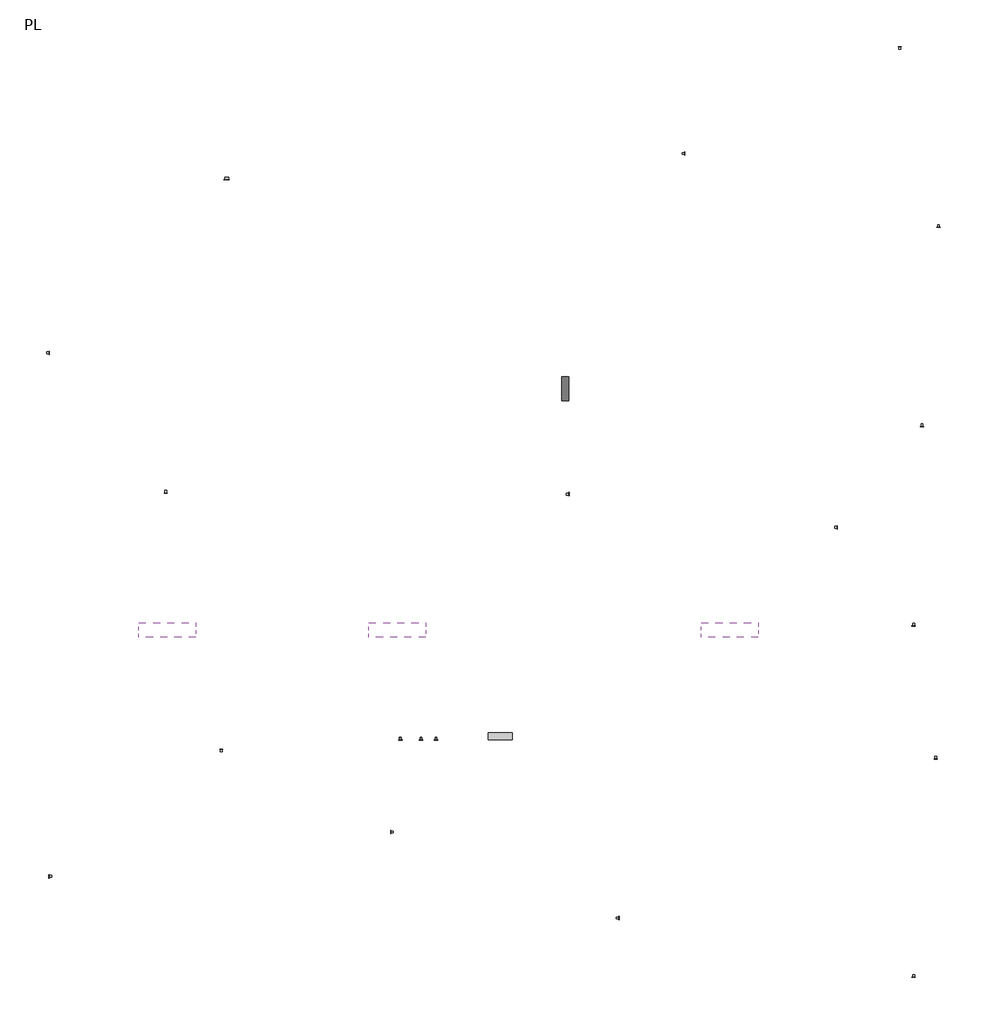
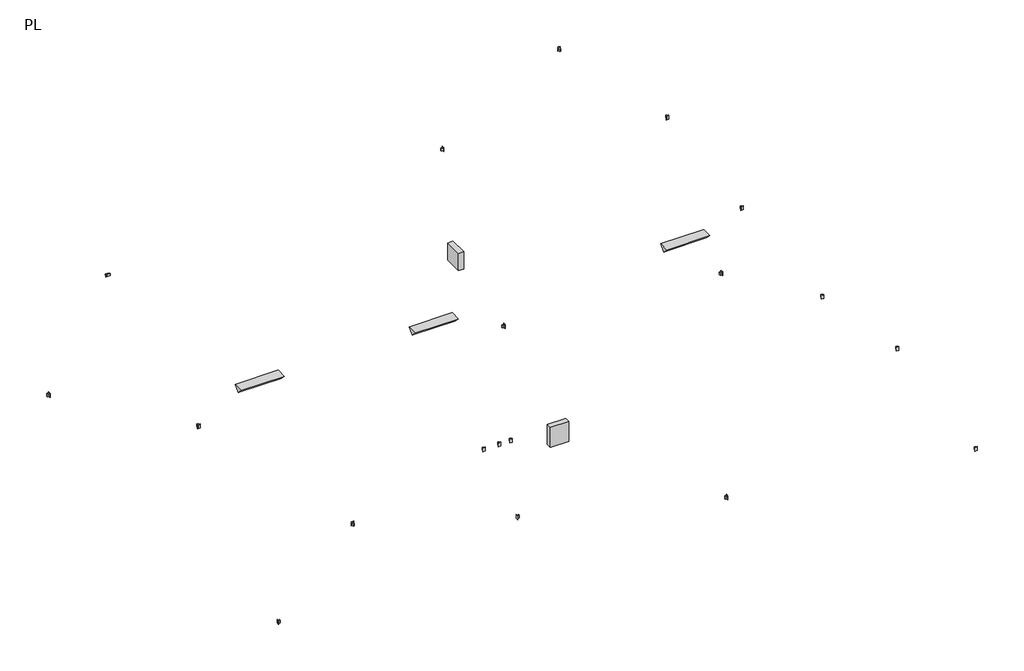
# One storey: 18 proxies, 3 light fixtures, 3 switching devices.
"""IFC4 building model written with IfcOpenShell, lengths in millimetres."""

import ifcopenshell
import ifcopenshell.guid

model = None  # the IFC model being written
_history = None  # IfcOwnerHistory: only IFC2X3 demands one
_inside = {}  # id of a spatial element -> (the spatial element, [elements in it])
_under = {}  # id of a project, library or spatial element -> (it, [spatial elements below it])
_declared = {}  # id of a project -> (the project, [libraries it declares])
_typed = {}  # id of a type object -> (the type object, [elements of that type])
_made_of = {}  # id of a material, layer set ... -> (it, [elements and type objects made of it])


def new_model(schema):
    """Start an empty IFC model of exactly this schema.

    Asked for "IFC4X3", IfcOpenShell would pick the latest addendum, in which some entities
    have other attributes; the version numbers below select the first issue.
    IFC2X3 requires an IfcOwnerHistory on every rooted entity: one is made here for all.
    """
    global model, _history
    if schema == "IFC4X3":
        model = ifcopenshell.file(schema_version=(4, 3, 0, 0))
    else:
        model = ifcopenshell.file(schema=schema)
    _inside.clear()
    _under.clear()
    _declared.clear()
    _typed.clear()
    _made_of.clear()
    _history = None
    if model.schema == "IFC2X3":
        org = make("IfcOrganization", Name="unknown")
        user = make(
            "IfcPersonAndOrganization",
            ThePerson=make("IfcPerson", FamilyName="unknown"),
            TheOrganization=org,
        )
        app = make(
            "IfcApplication",
            ApplicationDeveloper=org,
            Version="unknown",
            ApplicationFullName="unknown",
            ApplicationIdentifier="unknown",
        )
        _history = make(
            "IfcOwnerHistory",
            OwningUser=user,
            OwningApplication=app,
            ChangeAction="ADDED",
            CreationDate=0,
        )
    return model


def make(cls, **values):
    """One entity of the class cls with the attributes given. An attribute that is None is left unset."""
    return model.create_entity(
        cls, **{name: value for name, value in values.items() if value is not None}
    )


def rooted(cls, **values):
    """An entity with a GlobalId (a new one), such as an element, a storey or a relation."""
    return make(cls, GlobalId=ifcopenshell.guid.new(), OwnerHistory=_history, **values)


def si_unit(unit_type, name, prefix=None):
    """IfcSIUnit, for example si_unit("LENGTHUNIT", "METRE", prefix="MILLI")."""
    return make("IfcSIUnit", UnitType=unit_type, Prefix=prefix, Name=name)


def assignment(units):
    """IfcUnitAssignment: the units of a project."""
    return None if units is None else make("IfcUnitAssignment", Units=units)


def point(xyz):
    """IfcCartesianPoint."""
    return None if xyz is None else make("IfcCartesianPoint", Coordinates=xyz)


def direction(xyz):
    """IfcDirection."""
    return None if xyz is None else make("IfcDirection", DirectionRatios=xyz)


def frame(location, z_axis=None, x_axis=None):
    """IfcAxis2Placement3D, a coordinate frame: its origin and axes. An axis left out is left unset."""
    return make(
        "IfcAxis2Placement3D",
        Location=point(location),
        Axis=direction(z_axis),
        RefDirection=direction(x_axis),
    )


def origin():
    """The frame at (0, 0, 0) with its axes left unset."""
    return frame((0.0, 0.0, 0.0))


def origin_with_axes():
    """The frame at (0, 0, 0) with the z axis (0, 0, 1) and the x axis (1, 0, 0) written out."""
    return frame((0.0, 0.0, 0.0), z_axis=(0.0, 0.0, 1.0), x_axis=(1.0, 0.0, 0.0))


def place(relative_to, where):
    """IfcLocalPlacement: puts the frame where relative to a parent placement (None: the world)."""
    return make(
        "IfcLocalPlacement", PlacementRelTo=relative_to, RelativePlacement=where
    )


def context(
    kind, dimensions, precision=None, world=None, true_north=None, identifier=None
):
    """IfcGeometricRepresentationContext, for example the 3D "Model" context."""
    return make(
        "IfcGeometricRepresentationContext",
        ContextIdentifier=identifier,
        ContextType=kind,
        CoordinateSpaceDimension=dimensions,
        Precision=precision,
        WorldCoordinateSystem=world,
        TrueNorth=true_north,
    )


def project(units=None, contexts=None):
    """IfcProject with its units and contexts."""
    return rooted(
        "IfcProject",
        Name="project",
        RepresentationContexts=contexts,
        UnitsInContext=assignment(units),
    )


def spatial(cls, under=None, at=None, **own):
    """A site, building, storey or space (cls), placed at a placement, below another one or the project."""
    s = rooted(cls, ObjectPlacement=at, **own)
    if under is not None:
        _under.setdefault(under.id(), (under, []))[1].append(s)
    return s


def polyline(points):
    """IfcPolyline through the points."""
    return make("IfcPolyline", Points=[point(p) for p in points])


def outline(outer, holes=None, kind="AREA"):
    """IfcArbitraryClosedProfileDef: a profile drawn as a closed curve; with holes, ...WithVoids."""
    if holes is None:
        return make("IfcArbitraryClosedProfileDef", ProfileType=kind, OuterCurve=outer)
    return make(
        "IfcArbitraryProfileDefWithVoids",
        ProfileType=kind,
        OuterCurve=outer,
        InnerCurves=holes,
    )


def extrude(swept, where, along, depth):
    """IfcExtrudedAreaSolid: the profile swept, set in the frame where, extruded along a direction by depth."""
    return make(
        "IfcExtrudedAreaSolid",
        SweptArea=swept,
        Position=where,
        ExtrudedDirection=direction(along),
        Depth=depth,
    )


def shape(context_of_items, identifier, shape_type, items):
    """IfcShapeRepresentation: the items that make up one representation, for example the "Body"."""
    return make(
        "IfcShapeRepresentation",
        ContextOfItems=context_of_items,
        RepresentationIdentifier=identifier,
        RepresentationType=shape_type,
        Items=items,
    )


def source(mapping_origin, context_of_items, identifier, shape_type, items):
    """IfcRepresentationMap: a shape defined once, which mapped items show again and again."""
    return make(
        "IfcRepresentationMap",
        MappingOrigin=mapping_origin,
        MappedRepresentation=shape(context_of_items, identifier, shape_type, items),
    )


def transform(
    local_origin,
    x_axis=None,
    y_axis=None,
    z_axis=None,
    scale=None,
    scale2=None,
    scale3=None,
    uniform=True,
):
    """IfcCartesianTransformationOperator3D, or its non-uniform kind. x_axis, y_axis, z_axis: its Axis1, 2, 3."""
    if uniform:
        return make(
            "IfcCartesianTransformationOperator3D",
            Axis1=direction(x_axis),
            Axis2=direction(y_axis),
            LocalOrigin=point(local_origin),
            Scale=scale,
            Axis3=direction(z_axis),
        )
    return make(
        "IfcCartesianTransformationOperator3DnonUniform",
        Axis1=direction(x_axis),
        Axis2=direction(y_axis),
        LocalOrigin=point(local_origin),
        Scale=scale,
        Axis3=direction(z_axis),
        Scale2=scale2,
        Scale3=scale3,
    )


def mapped(mapping_source, mapping_target):
    """IfcMappedItem: shows the shape of a source again, moved by a transform."""
    return make(
        "IfcMappedItem", MappingSource=mapping_source, MappingTarget=mapping_target
    )


def made_of(thing, what):
    """Note that an element or type object is made of a material, layer set ...; save() writes the relation."""
    if what is not None:
        _made_of.setdefault(what.id(), (what, []))[1].append(thing)
    return thing


def element(
    cls,
    number,
    at=None,
    inside=None,
    cuts=None,
    type_object=None,
    material=None,
    context=None,
    identifier="Body",
    shape_type=None,
    held_by="IfcProductDefinitionShape",
    body=None,
    shapes=None,
    **own,
):
    """One element of the class cls, such as IfcWall. Its Tag is "e" and its number.

    at: its placement. inside: the storey or other place that contains it. cuts: it is an
    opening in that element (IfcRelVoidsElement). A single representation is given by context,
    identifier, shape_type and body (its items); several are given by shapes. held_by: the class
    of the entity that holds the representations. save() writes the other relations.
    """
    e = rooted(cls, Tag="e%d" % number, ObjectPlacement=at, **own)
    if body is not None:
        shapes = [shape(context, identifier, shape_type, body)]
    if shapes is not None:
        e.Representation = make(held_by, Representations=shapes)
    if inside is not None:
        _inside.setdefault(inside.id(), (inside, []))[1].append(e)
    if cuts is not None:
        rooted(
            "IfcRelVoidsElement", RelatingBuildingElement=cuts, RelatedOpeningElement=e
        )
    if type_object is not None:
        _typed.setdefault(type_object.id(), (type_object, []))[1].append(e)
    return made_of(e, material)


def aggregate(whole, parts):
    """IfcRelAggregates: a whole, such as a stair, and the parts it consists of."""
    return rooted("IfcRelAggregates", RelatingObject=whole, RelatedObjects=parts)


def save(model, path):
    """Write the relations noted so far, then the file.

    IfcRelAggregates (storeys below a building ...), IfcRelContainedInSpatialStructure (elements
    in a storey), IfcRelDefinesByType, IfcRelAssociatesMaterial and IfcRelDeclares: one each for
    every whole, place, type object, material and project.
    """
    for whole, parts in _under.values():
        aggregate(whole, parts)
    for where, things in _inside.values():
        rooted(
            "IfcRelContainedInSpatialStructure",
            RelatedElements=things,
            RelatingStructure=where,
        )
    for kind, things in _typed.values():
        rooted("IfcRelDefinesByType", RelatedObjects=things, RelatingType=kind)
    for what, things in _made_of.values():
        rooted("IfcRelAssociatesMaterial", RelatedObjects=things, RelatingMaterial=what)
    for by, libraries in _declared.values():
        rooted("IfcRelDeclares", RelatingContext=by, RelatedDefinitions=libraries)
    model.write(path)


def m_duplex_receptacle_standard_10251bba(model_context):
    return source(origin(), model_context, "Body", "SweptSolid", [
        extrude(outline(polyline([(19.05, 38.1), (19.05, -38.1), (-19.05, -38.1), (-19.05, 38.1), (19.05, 38.1)])), frame((0.0, 0.0, -53.975), z_axis=(0.0, 0.0, 1.0), x_axis=(1.0, 0.0, 0.0)), (0.0, 0.0, 1.0), 53.975),
        extrude(outline(polyline([(34.925, 57.15), (34.925, -57.15), (-34.925, -57.15), (-34.925, 57.15), (34.925, 57.15)])), origin_with_axes(), (0.0, 0.0, 1.0), 4.7625),
    ])


def m_lighting_and_appliance_panelboard_208v_mcb_100_a_1c5cc82c(model_context):
    return source(origin(), model_context, "Body", "SweptSolid", [
        extrude(outline(polyline([(349.2594706, 55.9943297), (349.2594706, -528.2056703), (-158.7405294, -528.2056703), (-158.7405294, 55.9943297), (349.2594706, 55.9943297)])), frame((0.0, 0.0, -146.1), z_axis=(0.0, 0.0, 1.0), x_axis=(1.0, 0.0, 0.0)), (0.0, 0.0, 1.0), 146.1),
    ])


def m_lighting_and_appliance_panelboard_208v_mlo_100_a_deb79597(model_context):
    return source(origin(), model_context, "Body", "SweptSolid", [
        extrude(outline(polyline([(254.0, -165.1), (254.0, -673.1), (-254.0, -673.1), (-254.0, -165.1), (254.0, -165.1)])), frame((0.0, 0.0, -146.1), z_axis=(0.0, 0.0, 1.0), x_axis=(1.0, 0.0, 0.0)), (0.0, 0.0, 1.0), 146.1),
    ])


def m_plain_recessed_lighting_fixture_300x1200_120_e46e8774(model_context):
    return source(origin(), model_context, "Body", "SweptSolid", [
        extrude(outline(polyline([(-300.0, 0.0), (0.0, 0.0), (-150.0, -150.0), (-300.0, 0.0)])), frame((0.0, 0.0, 0.0), z_axis=(1.0, 0.0, 0.0), x_axis=(0.0, 1.0, 0.0)), (0.0, 0.0, 1.0), 1200.0),
    ])


model = new_model("IFC4")

# Units and contexts
model_context = context("Model", 3, world=origin())
ifc_project = project(units=[si_unit("LENGTHUNIT", "METRE", prefix="MILLI")], contexts=[model_context])

# Site, building, storey
site = spatial("IfcSite", under=ifc_project)
building = spatial("IfcBuilding", under=site)
storey = spatial("IfcBuildingStorey", under=building, Name="PL", Elevation=500.0)

# Proxies
placement = place(None, origin())
m_duplex_receptacle_standard_shape = m_duplex_receptacle_standard_10251bba(model_context)
element("IfcBuildingElementProxy", 1, Name="M_Duplex Receptacle : Standard", ObjectType="M_Duplex Receptacle : Standard", at=placement, inside=storey, context=model_context, shape_type="MappedRepresentation", body=[
    mapped(m_duplex_receptacle_standard_shape, transform((-11924.1082979, -105.8587328, 960.0), x_axis=(1.0, 0.0, 0.0), y_axis=(0.0, 0.0, 1.0), z_axis=(0.0, -1.0, 0.0))),
])
element("IfcBuildingElementProxy", 2, Name="M_Duplex Receptacle : Standard", ObjectType="M_Duplex Receptacle : Standard", at=placement, inside=storey, context=model_context, shape_type="MappedRepresentation", body=[
    mapped(m_duplex_receptacle_standard_shape, transform((-10757.1359856, -5505.8587328, 960.0), x_axis=(-1.0, 0.0, 0.0), y_axis=(0.0, 0.0, 1.0), z_axis=(0.0, 1.0, 0.0))),
])
element("IfcBuildingElementProxy", 3, Name="M_Duplex Receptacle : Standard", ObjectType="M_Duplex Receptacle : Standard", at=placement, inside=storey, context=model_context, shape_type="MappedRepresentation", body=[
    mapped(m_duplex_receptacle_standard_shape, transform((-14381.6781998, -8181.5416269, 960.0), x_axis=(0.0, -1.0, 0.0), y_axis=(0.0, 0.0, 1.0), z_axis=(-1.0, 0.0, 0.0))),
])
element("IfcBuildingElementProxy", 4, Name="M_Duplex Receptacle : Standard", ObjectType="M_Duplex Receptacle : Standard", at=placement, inside=storey, context=model_context, shape_type="MappedRepresentation", body=[
    mapped(m_duplex_receptacle_standard_shape, transform((2218.3218002, -829.616059, 960.0), x_axis=(0.0, 1.0, 0.0), y_axis=(0.0, 0.0, 1.0), z_axis=(1.0, 0.0, 0.0))),
])
element("IfcBuildingElementProxy", 5, Name="M_Duplex Receptacle : Standard", ObjectType="M_Duplex Receptacle : Standard", at=placement, inside=storey, context=model_context, shape_type="MappedRepresentation", body=[
    mapped(m_duplex_receptacle_standard_shape, transform((-14381.6781998, 2846.3467249, 960.0), x_axis=(0.0, -1.0, 0.0), y_axis=(0.0, 0.0, -1.0), z_axis=(1.0, 0.0, 0.0))),
])
element("IfcBuildingElementProxy", 6, Name="M_Duplex Receptacle : Standard", ObjectType="M_Duplex Receptacle : Standard", at=placement, inside=storey, context=model_context, shape_type="MappedRepresentation", body=[
    mapped(m_duplex_receptacle_standard_shape, transform((4355.1554595, 5494.1412672, 960.0), x_axis=(1.0, 0.0, 0.0), y_axis=(0.0, 0.0, 1.0), z_axis=(0.0, -1.0, 0.0))),
])
element("IfcBuildingElementProxy", 7, Name="M_Duplex Receptacle : Standard", ObjectType="M_Duplex Receptacle : Standard", at=placement, inside=storey, context=model_context, shape_type="MappedRepresentation", body=[
    mapped(m_duplex_receptacle_standard_shape, transform((3538.2748408, 9294.1412672, 960.0), x_axis=(-1.0, 0.0, 0.0), y_axis=(0.0, 0.0, 1.0), z_axis=(0.0, 1.0, 0.0))),
])
element("IfcBuildingElementProxy", 8, Name="M_Duplex Receptacle : Standard", ObjectType="M_Duplex Receptacle : Standard", at=placement, inside=storey, context=model_context, shape_type="MappedRepresentation", body=[
    mapped(m_duplex_receptacle_standard_shape, transform((3830.0179189, -2905.8587328, 960.0), x_axis=(1.0, 0.0, 0.0), y_axis=(0.0, 0.0, 1.0), z_axis=(0.0, -1.0, 0.0))),
])
element("IfcBuildingElementProxy", 9, Name="M_Duplex Receptacle : Standard", ObjectType="M_Duplex Receptacle : Standard", at=placement, inside=storey, context=model_context, shape_type="MappedRepresentation", body=[
    mapped(m_duplex_receptacle_standard_shape, transform((4005.0637658, 1294.1412672, 960.0), x_axis=(1.0, 0.0, 0.0), y_axis=(0.0, 0.0, 1.0), z_axis=(0.0, -1.0, 0.0))),
])
element("IfcBuildingElementProxy", 10, Name="M_Duplex Receptacle : Standard", ObjectType="M_Duplex Receptacle : Standard", at=placement, inside=storey, context=model_context, shape_type="MappedRepresentation", body=[
    mapped(m_duplex_receptacle_standard_shape, transform((4296.8068439, -5705.8587328, 960.0), x_axis=(1.0, 0.0, 0.0), y_axis=(0.0, 0.0, 1.0), z_axis=(0.0, -1.0, 0.0))),
])
element("IfcBuildingElementProxy", 11, Name="M_Duplex Receptacle : Standard", ObjectType="M_Duplex Receptacle : Standard", at=placement, inside=storey, context=model_context, shape_type="MappedRepresentation", body=[
    mapped(m_duplex_receptacle_standard_shape, transform((3830.0179189, -10305.8587328, 960.0), x_axis=(1.0, 0.0, 0.0), y_axis=(0.0, 0.0, 1.0), z_axis=(0.0, -1.0, 0.0))),
])
element("IfcBuildingElementProxy", 12, Name="M_Duplex Receptacle : Standard", ObjectType="M_Duplex Receptacle : Standard", at=placement, inside=storey, context=model_context, shape_type="MappedRepresentation", body=[
    mapped(m_duplex_receptacle_standard_shape, transform((-2381.6781998, -9056.7708611, 960.0), x_axis=(0.0, -1.0, 0.0), y_axis=(0.0, 0.0, -1.0), z_axis=(1.0, 0.0, 0.0))),
])
element("IfcBuildingElementProxy", 13, Name="M_Duplex Receptacle : Standard", ObjectType="M_Duplex Receptacle : Standard", at=placement, inside=storey, context=model_context, shape_type="MappedRepresentation", body=[
    mapped(m_duplex_receptacle_standard_shape, transform((-7181.6781998, -7247.963777, 960.0), x_axis=(0.0, -1.0, 0.0), y_axis=(0.0, 0.0, 1.0), z_axis=(-1.0, 0.0, 0.0))),
])
element("IfcBuildingElementProxy", 14, Name="M_Duplex Receptacle : Standard", ObjectType="M_Duplex Receptacle : Standard", at=placement, inside=storey, context=model_context, shape_type="MappedRepresentation", body=[
    mapped(m_duplex_receptacle_standard_shape, transform((-10640.4387543, 6494.1412672, 960.0), x_axis=(0.0, 0.0, 1.0), y_axis=(-1.0, 0.0, 0.0), z_axis=(0.0, -1.0, 0.0))),
])
element("IfcBuildingElementProxy", 15, Name="M_Duplex Receptacle : Standard", ObjectType="M_Duplex Receptacle : Standard", at=placement, inside=storey, context=model_context, shape_type="MappedRepresentation", body=[
    mapped(m_duplex_receptacle_standard_shape, transform((-991.6781998, 7047.4470494, 960.0), x_axis=(0.0, 1.0, 0.0), y_axis=(0.0, 0.0, 1.0), z_axis=(1.0, 0.0, 0.0))),
])
element("IfcBuildingElementProxy", 16, Name="M_Duplex Receptacle : Standard", ObjectType="M_Duplex Receptacle : Standard", at=placement, inside=storey, context=model_context, shape_type="MappedRepresentation", body=[
    mapped(m_duplex_receptacle_standard_shape, transform((-3431.6781998, -129.4326716, 960.0), x_axis=(0.0, 1.0, 0.0), y_axis=(0.0, 0.0, 1.0), z_axis=(1.0, 0.0, 0.0))),
])
m_lighting_and_appliance_panelboard_208v_mcb_100_a_shape = m_lighting_and_appliance_panelboard_208v_mcb_100_a_1c5cc82c(model_context)
element("IfcBuildingElementProxy", 17, Name="M_Lighting and Appliance Panelboard - 208V MCB : 100 A", ObjectType="M_Lighting and Appliance Panelboard - 208V MCB : 100 A", at=placement, inside=storey, context=model_context, shape_type="MappedRepresentation", body=[
    mapped(m_lighting_and_appliance_panelboard_208v_mcb_100_a_shape, transform((-4974.3445292, -5305.8587328, 1644.0056703), x_axis=(1.0, 0.0, 0.0), y_axis=(0.0, 0.0, 1.0), z_axis=(0.0, -1.0, 0.0))),
])
m_lighting_and_appliance_panelboard_208v_mlo_100_a_shape = m_lighting_and_appliance_panelboard_208v_mlo_100_a_deb79597(model_context)
element("IfcBuildingElementProxy", 18, Name="M_Lighting and Appliance Panelboard - 208V MLO : 100 A", ObjectType="M_Lighting and Appliance Panelboard - 208V MLO : 100 A", at=placement, inside=storey, context=model_context, shape_type="MappedRepresentation", body=[
    mapped(m_lighting_and_appliance_panelboard_208v_mlo_100_a_shape, transform((-3431.6781998, 2087.8147219, 2119.1), x_axis=(0.0, 1.0, 0.0), y_axis=(0.0, 0.0, 1.0), z_axis=(1.0, 0.0, 0.0))),
])

# Light fixtures
m_plain_recessed_lighting_fixture_300x1200_120_shape = m_plain_recessed_lighting_fixture_300x1200_120_e46e8774(model_context)
element("IfcLightFixture", 19, ObjectType="M_Plain Recessed Lighting Fixture : 300x1200 - 120", at=placement, inside=storey, context=model_context, shape_type="MappedRepresentation", body=[
    mapped(m_plain_recessed_lighting_fixture_300x1200_120_shape, transform((-7647.9902357, -2843.9180174, 4050.0), x_axis=(1.0, 0.0, 0.0), y_axis=(0.0, 1.0, 0.0), z_axis=(0.0, 0.0, 1.0))),
])
element("IfcLightFixture", 20, ObjectType="M_Plain Recessed Lighting Fixture : 300x1200 - 120", at=placement, inside=storey, context=model_context, shape_type="MappedRepresentation", body=[
    mapped(m_plain_recessed_lighting_fixture_300x1200_120_shape, transform((-646.1563616, -2843.9180174, 4050.0), x_axis=(1.0, 0.0, 0.0), y_axis=(0.0, 1.0, 0.0), z_axis=(0.0, 0.0, 1.0))),
])
element("IfcLightFixture", 21, ObjectType="M_Plain Recessed Lighting Fixture : 300x1200 - 120", at=placement, inside=storey, context=model_context, shape_type="MappedRepresentation", body=[
    mapped(m_plain_recessed_lighting_fixture_300x1200_120_shape, transform((-12490.925332, -2843.9180174, 4050.0), x_axis=(1.0, 0.0, 0.0), y_axis=(0.0, 1.0, 0.0), z_axis=(0.0, 0.0, 1.0))),
])

# Switching devices
element("IfcSwitchingDevice", 22, ObjectType="M_Lighting Switches : Three Way", at=placement, inside=storey, context=model_context, shape_type="MappedRepresentation", body=[
    mapped(m_duplex_receptacle_standard_shape, transform((-6981.9346231, -5305.8587328, 1700.0), x_axis=(1.0, 0.0, 0.0), y_axis=(0.0, 0.0, 1.0), z_axis=(0.0, -1.0, 0.0))),
])
element("IfcSwitchingDevice", 23, ObjectType="M_Lighting Switches : Three Way", at=placement, inside=storey, context=model_context, shape_type="MappedRepresentation", body=[
    mapped(m_duplex_receptacle_standard_shape, transform((-6549.1043357, -5305.8587328, 1700.0), x_axis=(1.0, 0.0, 0.0), y_axis=(0.0, 0.0, 1.0), z_axis=(0.0, -1.0, 0.0))),
])
element("IfcSwitchingDevice", 24, ObjectType="M_Lighting Switches : Three Way", at=placement, inside=storey, context=model_context, shape_type="MappedRepresentation", body=[
    mapped(m_duplex_receptacle_standard_shape, transform((-6232.8369052, -5305.8587328, 1700.0), x_axis=(1.0, 0.0, 0.0), y_axis=(0.0, 0.0, 1.0), z_axis=(0.0, -1.0, 0.0))),
])

save(model, "model.ifc")

# Revit data of these elements
# Project information
#   Project Issue Date = "Issue Date"
#   Project Status = "Project Status"
#   Client Name = "Owner"
#   Project Address = "Enter address here"
#   Project Name = "Project Name"
#   Project Number = "Project Number"
# Type "M_Duplex Receptacle : Standard"
#   Label = ""
#   Switch Voltage = 120 V
#   Load = 180 VA
#   Default Elevation = 460 mm
#   Load Classification = Receptacle
#   Assembly Code = ""
# Type "M_Lighting and Appliance Panelboard - 208V MCB : 100 A"
#   built-in parameter 1140081 [instance default] = "Recessed"
#   built-in parameter 1140083 [instance default] = "Type 1"
#   Width = 508 mm
#   built-in parameter 1140082 [instance default] = 100 (stored number, unit not read)
#   built-in parameter 1140140 = 100 (stored number, unit not read)
#   Height [instance default] = 584.2 mm
#   Depth = 146.1 mm
#   Default Elevation = 1200 mm
#   42 Circuit Height = 1270 mm
#   30 Circuit Height = 736.6 mm
#   24 Circuit Height = 660.4 mm
#   12 Circuit Height = 584.2 mm
#   built-in parameter 1140079 [instance default] = 12
#   Load Classification = Other
# Type "M_Lighting and Appliance Panelboard - 208V MLO : 100 A"
#   built-in parameter 1140081 [instance default] = "Recessed"
#   built-in parameter 1140083 [instance default] = "Type 1"
#   Width = 508 mm
#   built-in parameter 1140082 [instance default] = 100 (stored number, unit not read)
#   Height [instance default] = 508 mm
#   Depth = 146.1 mm
#   Default Elevation = 1200 mm
#   42 Circuit Height = 1041.4 mm
#   30 Circuit Height = 660.4 mm
#   24 Circuit Height = 584.2 mm
#   12 Circuit Height = 508 mm
#   built-in parameter 1140079 [instance default] = 12
#   Load Classification = Other
# Type "M_Plain Recessed Lighting Fixture : 300x1200 - 120"
#   Photometric Web File = "1x42A12.ies"
#   Width = 300 mm
#   Wattage = 64 W
#   built-in parameter 1150110 = 1 (stored number, unit not read)
#   built-in parameter 1150109 = 1 (stored number, unit not read)
#   built-in parameter 1150113 = 1 (stored number, unit not read)
#   Tilt Angle = -90.00°
#   Lumens = 5699.84 lm
#   built-in parameter 1114217 = 0.88 (stored number, unit not read)
#   built-in parameter 1150115 = 1 (stored number, unit not read)
#   built-in parameter 1150105 = 453.579 (stored number, unit not read)
#   Length = 1200 mm
#   built-in parameter 1150112 = 1 (stored number, unit not read)
#   built-in parameter 1150114 = 1 (stored number, unit not read)
#   built-in parameter 1150107 = 4230 (stored number, unit not read)
#   built-in parameter 1150106 = 4.53579 (stored number, unit not read)
#   Emit from Rectangle Width = 300 mm
#   Emit from Rectangle Length = 1200 mm
#   built-in parameter 1150104 = 8.27394 (stored number, unit not read)
#   Depth = 150 mm
#   Default Elevation = 2000 mm
#   Ballast Voltage = 120 V
#   built-in parameter 1114218 = 0.88 (stored number, unit not read)
#   built-in parameter 1150133 = 10 (stored number, unit not read)
#   Apparent Load = 64 VA
#   built-in parameter 1150134 = 8
#   built-in parameter 1150137 = 1
#   Color Filter = 16777215
#   built-in parameter 1140040 [instance default] = 1
#   Load Classification = Lighting - Dwelling Unit
#   Emit Shape Visible in Rendering = no
#   Dimming Lamp Color Temperature Shift = (empty or 0)
#   Assembly Code = ""
# Type "M_Lighting Switches : Three Way"
#   Label = "3"
#   Switch Voltage [instance default] = 120 V
#   Default Elevation = 1200 mm
#   Apparent Load = 0 VA
#   Load Classification = Other
#   Assembly Code = ""
# Element 1 (IfcBuildingElementProxy, "M_Duplex Receptacle : Standard")
#   Mark = "2"
#   Phase Created = New Construction
# Element 2 (IfcBuildingElementProxy, "M_Duplex Receptacle : Standard")
#   Mark = "3"
#   Phase Created = New Construction
# Element 3 (IfcBuildingElementProxy, "M_Duplex Receptacle : Standard")
#   Mark = "4"
#   Phase Created = New Construction
# Element 4 (IfcBuildingElementProxy, "M_Duplex Receptacle : Standard")
#   Mark = "5"
#   Phase Created = New Construction
# Element 5 (IfcBuildingElementProxy, "M_Duplex Receptacle : Standard")
#   Mark = "7"
#   Phase Created = New Construction
# Element 6 (IfcBuildingElementProxy, "M_Duplex Receptacle : Standard")
#   Mark = "8"
#   Phase Created = New Construction
# Element 7 (IfcBuildingElementProxy, "M_Duplex Receptacle : Standard")
#   Mark = "9"
#   Phase Created = New Construction
# Element 8 (IfcBuildingElementProxy, "M_Duplex Receptacle : Standard")
#   Mark = "10"
#   Phase Created = New Construction
# Element 9 (IfcBuildingElementProxy, "M_Duplex Receptacle : Standard")
#   Mark = "11"
#   Phase Created = New Construction
# Element 10 (IfcBuildingElementProxy, "M_Duplex Receptacle : Standard")
#   Mark = "12"
#   Phase Created = New Construction
# Element 11 (IfcBuildingElementProxy, "M_Duplex Receptacle : Standard")
#   Mark = "13"
#   Phase Created = New Construction
# Element 12 (IfcBuildingElementProxy, "M_Duplex Receptacle : Standard")
#   Mark = "14"
#   Phase Created = New Construction
# Element 13 (IfcBuildingElementProxy, "M_Duplex Receptacle : Standard")
#   Mark = "15"
#   Phase Created = New Construction
# Element 14 (IfcBuildingElementProxy, "M_Duplex Receptacle : Standard")
#   Mark = "16"
#   Phase Created = New Construction
# Element 15 (IfcBuildingElementProxy, "M_Duplex Receptacle : Standard")
#   Mark = "17"
#   Phase Created = New Construction
# Element 16 (IfcBuildingElementProxy, "M_Duplex Receptacle : Standard")
#   Mark = "18"
#   Phase Created = New Construction
# Element 17 (IfcBuildingElementProxy, "M_Lighting and Appliance Panelboard - 208V MCB : 100 A")
#   Mark = "2"
#   built-in parameter 1140081 = "Recessed"
#   built-in parameter 1140083 = "Type 1"
#   built-in parameter 1140082 = 100 (stored number, unit not read)
#   Height = 584.2 mm
#   built-in parameter 1140079 = 12
#   built-in parameter 1140064 = 120/208 Wye
#   Phase Created = New Construction
# Element 18 (IfcBuildingElementProxy, "M_Lighting and Appliance Panelboard - 208V MLO : 100 A")
#   Mark = "1"
#   built-in parameter 1140081 = "Recessed"
#   built-in parameter 1140083 = "Type 1"
#   built-in parameter 1140082 = 100 (stored number, unit not read)
#   Height = 508 mm
#   built-in parameter 1140079 = 12
#   built-in parameter 1140064 = 120/208 Wye
#   Phase Created = New Construction
# Element 19 (IfcLightFixture, "M_Plain Recessed Lighting Fixture : 300x1200 - 120")
#   Mark = "1"
#   built-in parameter 1140040 = 1
#   Phase Created = New Construction
# Element 20 (IfcLightFixture, "M_Plain Recessed Lighting Fixture : 300x1200 - 120")
#   Mark = "2"
#   built-in parameter 1140040 = 1
#   Phase Created = New Construction
# Element 21 (IfcLightFixture, "M_Plain Recessed Lighting Fixture : 300x1200 - 120")
#   Mark = "3"
#   built-in parameter 1140040 = 1
#   Phase Created = New Construction
# Element 22 (IfcSwitchingDevice, "M_Lighting Switches : Three Way")
#   Mark = "1"
#   Switch Voltage = 120 V
#   Phase Created = New Construction
# Element 23 (IfcSwitchingDevice, "M_Lighting Switches : Three Way")
#   Mark = "2"
#   Switch Voltage = 120 V
#   Phase Created = New Construction
# Element 24 (IfcSwitchingDevice, "M_Lighting Switches : Three Way")
#   Mark = "3"
#   Switch Voltage = 120 V
#   Phase Created = New Construction
